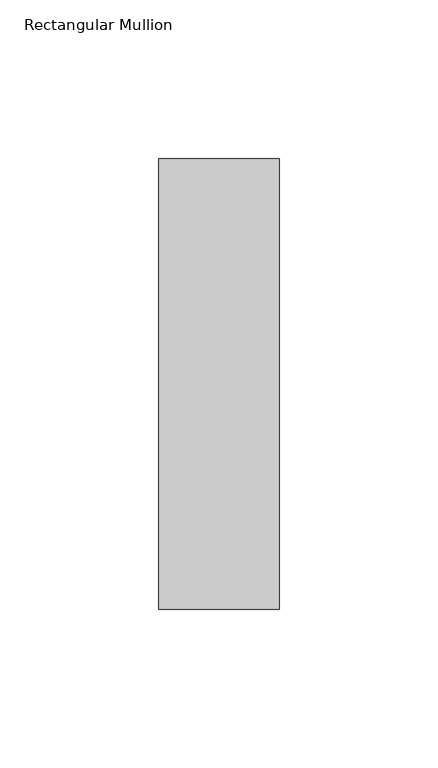
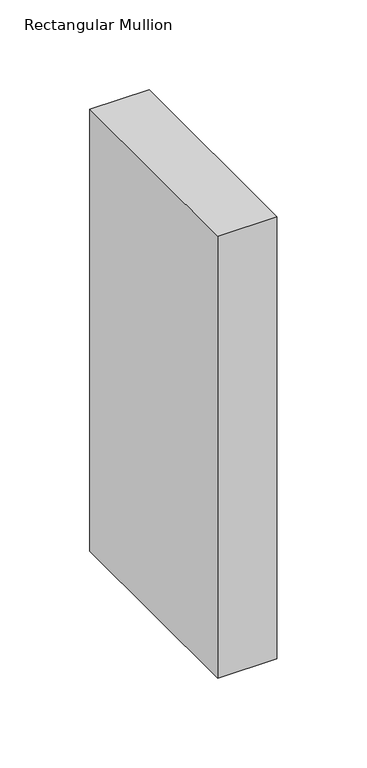
"""IFC4 building model written with IfcOpenShell, lengths in millimetres: member geometry, Rectangular Mullion : NLRS_21_CWM_hsb-regel 38x142_gen_rsf."""

from ifc_helpers import new_model, si_unit, frame, origin, place, context, project, spatial, polyline, outline, extrude, source, transform, mapped, element, save


def rectangular_mullion_8803486b(model_context):
    return source(origin(), model_context, "Body", "SweptSolid", [
        extrude(outline(polyline([(0.0, -71.0), (-38.0, -71.0), (-38.0, 71.0), (0.0, 71.0), (0.0, -71.0)])), frame((0.0, 0.0, -300.0), z_axis=(0.0, 0.0, 1.0), x_axis=(1.0, 0.0, 0.0)), (0.0, 0.0, 1.0), 300.0),
    ])


if __name__ == "__main__":
    model = new_model("IFC4")
    model_context = context("Model", 3, world=origin())
    ifc_project = project(units=[si_unit("LENGTHUNIT", "METRE", prefix="MILLI")], contexts=[model_context])
    site = spatial("IfcSite", under=ifc_project)
    building = spatial("IfcBuilding", under=site)
    placement = place(None, origin())
    rectangular_mullion_shape = rectangular_mullion_8803486b(model_context)
    element("IfcMember", 1, ObjectType="Rectangular Mullion : NLRS_21_CWM_hsb-regel 38x142_gen_rsf", at=placement, inside=building, context=model_context, shape_type="MappedRepresentation", body=[
        mapped(rectangular_mullion_shape, transform((0.0, 0.0, 0.0), x_axis=(1.0, 0.0, 0.0), y_axis=(0.0, 1.0, 0.0), z_axis=(0.0, 0.0, 1.0))),
    ])
    save(model, "model.ifc")

# Revit data of these elements
# Type "Rectangular Mullion : NLRS_21_CWM_hsb-regel 38x142_gen_rsf"
#   Export Type to IFC As = "IfcWall"
#   Type IfcGUID = "07M7mRoiH1CR8m_RSKIwpF"
#   Assembly Code = "21.10"
#   built-in parameter 1007322 = 0.465879 (stored number, unit not read)
#   built-in parameter 1007321 = 0.062336 (stored number, unit not read)
#   built-in parameter 1007320 = 0.062336 (stored number, unit not read)
# Element 1 (IfcMember, "Rectangular Mullion : NLRS_21_CWM_hsb-regel 38x142_gen_rsf")
#   Materials on its faces: "NLRS_i2_hout naaldhout vuren_gen_rsf"
# Materials
#   "NLRS_i2_hout naaldhout vuren_gen_rsf": class "I - Hout", colour RGB 234 199 147, transparency 0, Keynote = "i2", Manufacturer = "Revit Standards Foundation", URL = "www.revitstandards.org", Description = "hout vuren", Cost = 0
